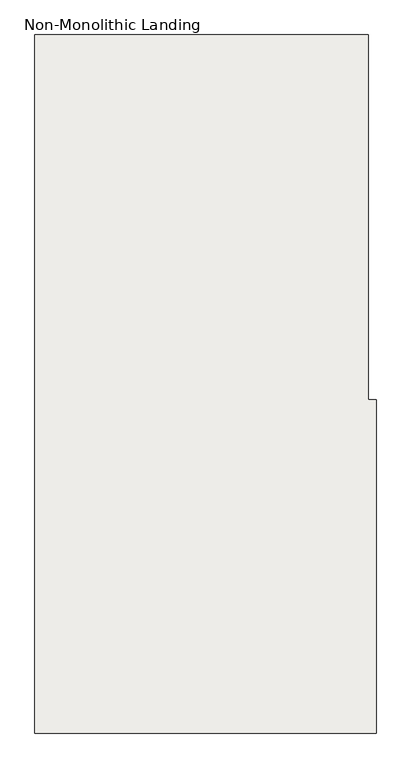
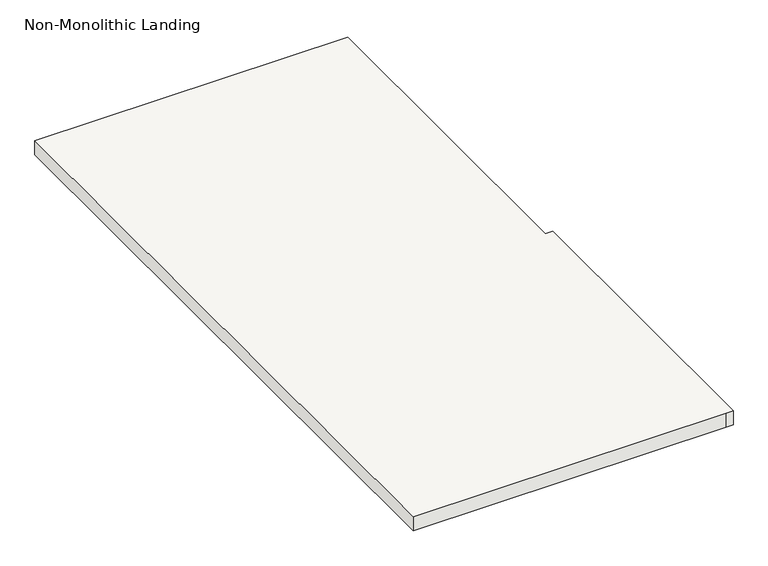
"""IFC4 building model written with IfcOpenShell, lengths in millimetres: slab geometry, Non-Monolithic Landing."""

from ifc_helpers import new_model, si_unit, origin, place, context, project, spatial, faceted_brep, source, transform, mapped, element, save


def non_monolithic_landing_fbd0f5ca(model_context):
    return source(origin(), model_context, "Body", "Brep", [
        faceted_brep([(663695.788677, -549416.0413841, 3069.4527027), (663721.188677, -549416.0413841, 3094.8527027), (663721.188677, -550482.8413841, 3094.8527027), (663695.788677, -550482.8413841, 3069.4527027), (662654.388677, -549416.0413841, 3113.9027027), (662654.388677, -551651.2413841, 3113.9027027), (663721.188677, -551651.2413841, 3113.9027027), (663746.588677, -551651.2413841, 3113.9027027), (663746.588677, -550584.4413841, 3113.9027027), (663721.188677, -550584.4413841, 3113.9027027), (663721.188677, -549416.0413841, 3113.9027027), (663695.788677, -550482.8413841, 3063.1027027), (663721.188677, -550482.8413841, 3063.1027027), (663721.188677, -550584.4413841, 3063.1027027), (663746.588677, -550584.4413841, 3063.1027027), (663746.588677, -551651.2413841, 3063.1027027), (663721.188677, -551651.2413841, 3063.1027027), (662654.388677, -551651.2413841, 3063.1027027), (662654.388677, -549416.0413841, 3063.1027027), (663695.788677, -549416.0413841, 3063.1027027)], [[[0, 1, 2, 3]], [[4, 5, 6, 7, 8, 9, 10]], [[11, 12, 13, 14, 15, 16, 17, 18, 19]], [[12, 11, 3, 2]], [[11, 19, 0, 3]], [[4, 10, 1, 0, 19, 18]], [[5, 4, 18, 17]], [[6, 5, 17, 16]], [[7, 6, 16, 15]], [[8, 7, 15, 14]], [[9, 8, 14, 13]], [[10, 9, 13, 12, 2, 1]]]),
    ])


if __name__ == "__main__":
    model = new_model("IFC4")
    model_context = context("Model", 3, world=origin())
    ifc_project = project(units=[si_unit("LENGTHUNIT", "METRE", prefix="MILLI")], contexts=[model_context])
    site = spatial("IfcSite", under=ifc_project)
    building = spatial("IfcBuilding", under=site)
    placement = place(None, origin())
    non_monolithic_landing_shape = non_monolithic_landing_fbd0f5ca(model_context)
    element("IfcSlab", 1, ObjectType="Non-Monolithic Landing", at=placement, inside=building, context=model_context, shape_type="MappedRepresentation", body=[
        mapped(non_monolithic_landing_shape, transform((0.0, 0.0, 0.0), x_axis=(1.0, 0.0, 0.0), y_axis=(0.0, 1.0, 0.0), z_axis=(0.0, 0.0, 1.0))),
    ])
    save(model, "model.ifc")
